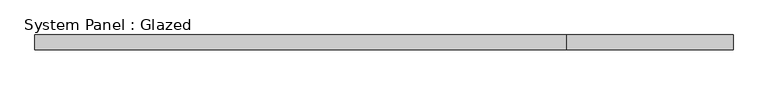
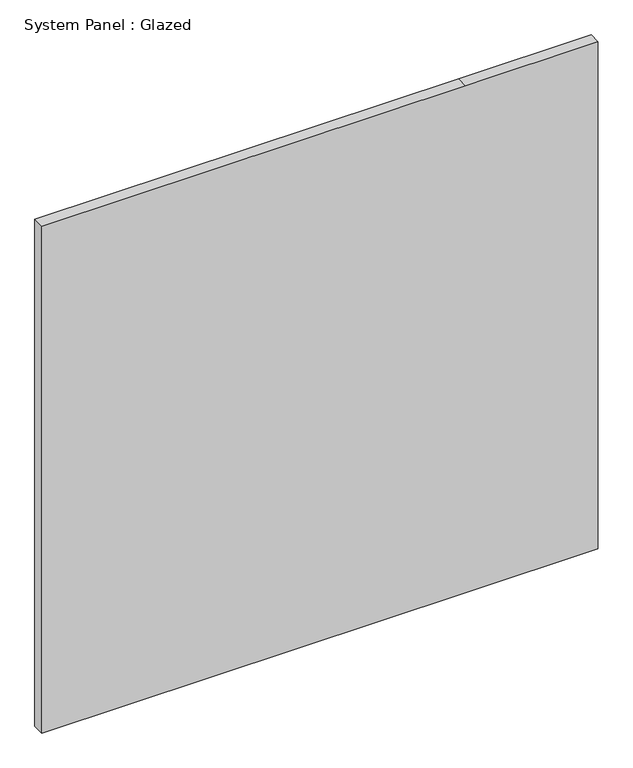
"""IFC4 building model written with IfcOpenShell, lengths in millimetres: plate geometry, System Panel : Glazed."""

import ifcopenshell
import ifcopenshell.guid

model = None  # the IFC model being written
_history = None  # IfcOwnerHistory: only IFC2X3 demands one
_inside = {}  # id of a spatial element -> (the spatial element, [elements in it])
_under = {}  # id of a project, library or spatial element -> (it, [spatial elements below it])
_declared = {}  # id of a project -> (the project, [libraries it declares])
_typed = {}  # id of a type object -> (the type object, [elements of that type])
_made_of = {}  # id of a material, layer set ... -> (it, [elements and type objects made of it])


def new_model(schema):
    """Start an empty IFC model of exactly this schema.

    Asked for "IFC4X3", IfcOpenShell would pick the latest addendum, in which some entities
    have other attributes; the version numbers below select the first issue.
    IFC2X3 requires an IfcOwnerHistory on every rooted entity: one is made here for all.
    """
    global model, _history
    if schema == "IFC4X3":
        model = ifcopenshell.file(schema_version=(4, 3, 0, 0))
    else:
        model = ifcopenshell.file(schema=schema)
    _inside.clear()
    _under.clear()
    _declared.clear()
    _typed.clear()
    _made_of.clear()
    _history = None
    if model.schema == "IFC2X3":
        org = make("IfcOrganization", Name="unknown")
        user = make(
            "IfcPersonAndOrganization",
            ThePerson=make("IfcPerson", FamilyName="unknown"),
            TheOrganization=org,
        )
        app = make(
            "IfcApplication",
            ApplicationDeveloper=org,
            Version="unknown",
            ApplicationFullName="unknown",
            ApplicationIdentifier="unknown",
        )
        _history = make(
            "IfcOwnerHistory",
            OwningUser=user,
            OwningApplication=app,
            ChangeAction="ADDED",
            CreationDate=0,
        )
    return model


def make(cls, **values):
    """One entity of the class cls with the attributes given. An attribute that is None is left unset."""
    return model.create_entity(
        cls, **{name: value for name, value in values.items() if value is not None}
    )


def rooted(cls, **values):
    """An entity with a GlobalId (a new one), such as an element, a storey or a relation."""
    return make(cls, GlobalId=ifcopenshell.guid.new(), OwnerHistory=_history, **values)


def si_unit(unit_type, name, prefix=None):
    """IfcSIUnit, for example si_unit("LENGTHUNIT", "METRE", prefix="MILLI")."""
    return make("IfcSIUnit", UnitType=unit_type, Prefix=prefix, Name=name)


def assignment(units):
    """IfcUnitAssignment: the units of a project."""
    return None if units is None else make("IfcUnitAssignment", Units=units)


def point(xyz):
    """IfcCartesianPoint."""
    return None if xyz is None else make("IfcCartesianPoint", Coordinates=xyz)


def direction(xyz):
    """IfcDirection."""
    return None if xyz is None else make("IfcDirection", DirectionRatios=xyz)


def frame(location, z_axis=None, x_axis=None):
    """IfcAxis2Placement3D, a coordinate frame: its origin and axes. An axis left out is left unset."""
    return make(
        "IfcAxis2Placement3D",
        Location=point(location),
        Axis=direction(z_axis),
        RefDirection=direction(x_axis),
    )


def origin():
    """The frame at (0, 0, 0) with its axes left unset."""
    return frame((0.0, 0.0, 0.0))


def place(relative_to, where):
    """IfcLocalPlacement: puts the frame where relative to a parent placement (None: the world)."""
    return make(
        "IfcLocalPlacement", PlacementRelTo=relative_to, RelativePlacement=where
    )


def context(
    kind, dimensions, precision=None, world=None, true_north=None, identifier=None
):
    """IfcGeometricRepresentationContext, for example the 3D "Model" context."""
    return make(
        "IfcGeometricRepresentationContext",
        ContextIdentifier=identifier,
        ContextType=kind,
        CoordinateSpaceDimension=dimensions,
        Precision=precision,
        WorldCoordinateSystem=world,
        TrueNorth=true_north,
    )


def project(units=None, contexts=None):
    """IfcProject with its units and contexts."""
    return rooted(
        "IfcProject",
        Name="project",
        RepresentationContexts=contexts,
        UnitsInContext=assignment(units),
    )


def spatial(cls, under=None, at=None, **own):
    """A site, building, storey or space (cls), placed at a placement, below another one or the project."""
    s = rooted(cls, ObjectPlacement=at, **own)
    if under is not None:
        _under.setdefault(under.id(), (under, []))[1].append(s)
    return s


def polyline(points):
    """IfcPolyline through the points."""
    return make("IfcPolyline", Points=[point(p) for p in points])


def outline(outer, holes=None, kind="AREA"):
    """IfcArbitraryClosedProfileDef: a profile drawn as a closed curve; with holes, ...WithVoids."""
    if holes is None:
        return make("IfcArbitraryClosedProfileDef", ProfileType=kind, OuterCurve=outer)
    return make(
        "IfcArbitraryProfileDefWithVoids",
        ProfileType=kind,
        OuterCurve=outer,
        InnerCurves=holes,
    )


def extrude(swept, where, along, depth):
    """IfcExtrudedAreaSolid: the profile swept, set in the frame where, extruded along a direction by depth."""
    return make(
        "IfcExtrudedAreaSolid",
        SweptArea=swept,
        Position=where,
        ExtrudedDirection=direction(along),
        Depth=depth,
    )


def shape(context_of_items, identifier, shape_type, items):
    """IfcShapeRepresentation: the items that make up one representation, for example the "Body"."""
    return make(
        "IfcShapeRepresentation",
        ContextOfItems=context_of_items,
        RepresentationIdentifier=identifier,
        RepresentationType=shape_type,
        Items=items,
    )


def source(mapping_origin, context_of_items, identifier, shape_type, items):
    """IfcRepresentationMap: a shape defined once, which mapped items show again and again."""
    return make(
        "IfcRepresentationMap",
        MappingOrigin=mapping_origin,
        MappedRepresentation=shape(context_of_items, identifier, shape_type, items),
    )


def transform(
    local_origin,
    x_axis=None,
    y_axis=None,
    z_axis=None,
    scale=None,
    scale2=None,
    scale3=None,
    uniform=True,
):
    """IfcCartesianTransformationOperator3D, or its non-uniform kind. x_axis, y_axis, z_axis: its Axis1, 2, 3."""
    if uniform:
        return make(
            "IfcCartesianTransformationOperator3D",
            Axis1=direction(x_axis),
            Axis2=direction(y_axis),
            LocalOrigin=point(local_origin),
            Scale=scale,
            Axis3=direction(z_axis),
        )
    return make(
        "IfcCartesianTransformationOperator3DnonUniform",
        Axis1=direction(x_axis),
        Axis2=direction(y_axis),
        LocalOrigin=point(local_origin),
        Scale=scale,
        Axis3=direction(z_axis),
        Scale2=scale2,
        Scale3=scale3,
    )


def mapped(mapping_source, mapping_target):
    """IfcMappedItem: shows the shape of a source again, moved by a transform."""
    return make(
        "IfcMappedItem", MappingSource=mapping_source, MappingTarget=mapping_target
    )


def made_of(thing, what):
    """Note that an element or type object is made of a material, layer set ...; save() writes the relation."""
    if what is not None:
        _made_of.setdefault(what.id(), (what, []))[1].append(thing)
    return thing


def element(
    cls,
    number,
    at=None,
    inside=None,
    cuts=None,
    type_object=None,
    material=None,
    context=None,
    identifier="Body",
    shape_type=None,
    held_by="IfcProductDefinitionShape",
    body=None,
    shapes=None,
    **own,
):
    """One element of the class cls, such as IfcWall. Its Tag is "e" and its number.

    at: its placement. inside: the storey or other place that contains it. cuts: it is an
    opening in that element (IfcRelVoidsElement). A single representation is given by context,
    identifier, shape_type and body (its items); several are given by shapes. held_by: the class
    of the entity that holds the representations. save() writes the other relations.
    """
    e = rooted(cls, Tag="e%d" % number, ObjectPlacement=at, **own)
    if body is not None:
        shapes = [shape(context, identifier, shape_type, body)]
    if shapes is not None:
        e.Representation = make(held_by, Representations=shapes)
    if inside is not None:
        _inside.setdefault(inside.id(), (inside, []))[1].append(e)
    if cuts is not None:
        rooted(
            "IfcRelVoidsElement", RelatingBuildingElement=cuts, RelatedOpeningElement=e
        )
    if type_object is not None:
        _typed.setdefault(type_object.id(), (type_object, []))[1].append(e)
    return made_of(e, material)


def aggregate(whole, parts):
    """IfcRelAggregates: a whole, such as a stair, and the parts it consists of."""
    return rooted("IfcRelAggregates", RelatingObject=whole, RelatedObjects=parts)


def save(model, path):
    """Write the relations noted so far, then the file.

    IfcRelAggregates (storeys below a building ...), IfcRelContainedInSpatialStructure (elements
    in a storey), IfcRelDefinesByType, IfcRelAssociatesMaterial and IfcRelDeclares: one each for
    every whole, place, type object, material and project.
    """
    for whole, parts in _under.values():
        aggregate(whole, parts)
    for where, things in _inside.values():
        rooted(
            "IfcRelContainedInSpatialStructure",
            RelatedElements=things,
            RelatingStructure=where,
        )
    for kind, things in _typed.values():
        rooted("IfcRelDefinesByType", RelatedObjects=things, RelatingType=kind)
    for what, things in _made_of.values():
        rooted("IfcRelAssociatesMaterial", RelatedObjects=things, RelatingMaterial=what)
    for by, libraries in _declared.values():
        rooted("IfcRelDeclares", RelatingContext=by, RelatedDefinitions=libraries)
    model.write(path)


def system_panel_glazed_70527e68(model_context):
    return source(origin(), model_context, "Body", "SweptSolid", [
        extrude(outline(polyline([(0.0, -600.075), (0.0, 314.325), (0.0, 600.075), (1155.7, 600.075), (1155.7, 314.325), (1155.7, -600.075), (0.0, -600.075)])), frame((0.0, -44.45, 0.0), z_axis=(0.0, 1.0, 0.0), x_axis=(0.0, 0.0, 1.0)), (0.0, 0.0, 1.0), 25.4),
    ])


if __name__ == "__main__":
    model = new_model("IFC4")
    model_context = context("Model", 3, world=origin())
    ifc_project = project(units=[si_unit("LENGTHUNIT", "METRE", prefix="MILLI")], contexts=[model_context])
    site = spatial("IfcSite", under=ifc_project)
    building = spatial("IfcBuilding", under=site)
    placement = place(None, origin())
    system_panel_glazed_shape = system_panel_glazed_70527e68(model_context)
    element("IfcPlate", 1, ObjectType="System Panel : Glazed", at=placement, inside=building, context=model_context, shape_type="MappedRepresentation", body=[
        mapped(system_panel_glazed_shape, transform((0.0, 0.0, 0.0), x_axis=(1.0, 0.0, 0.0), y_axis=(0.0, 1.0, 0.0), z_axis=(0.0, 0.0, 1.0))),
    ])
    save(model, "model.ifc")

# Revit data of these elements
# Type "System Panel : Glazed"
#   Construction Type Id = "GSP4R"
#   Analytic Construction = "1/8 in Pilkington single glazing"
#   Visual Light Transmittance = 0.9
#   Solar Heat Gain Coefficient = 0.86
#   Heat Transfer Coefficient (U) = 1.18115 BTU/(h·ft²·°F)
#   Define Thermal Properties by = 1
# Element 1 (IfcPlate, "System Panel : Glazed")
#   Materials on its faces: "Glass"
# Materials
#   "Glass": class "Glass", colour RGB 0 128 192, transparency 0.75, Description = "Soda Lime Glass", Cost = 0
